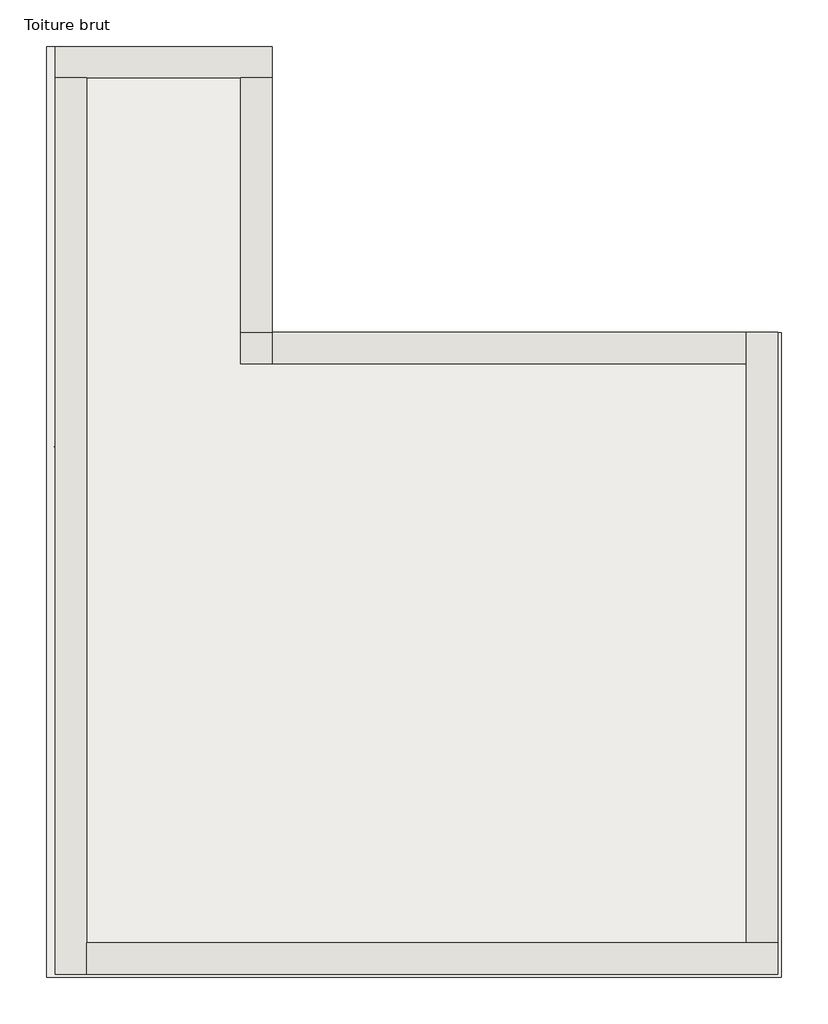
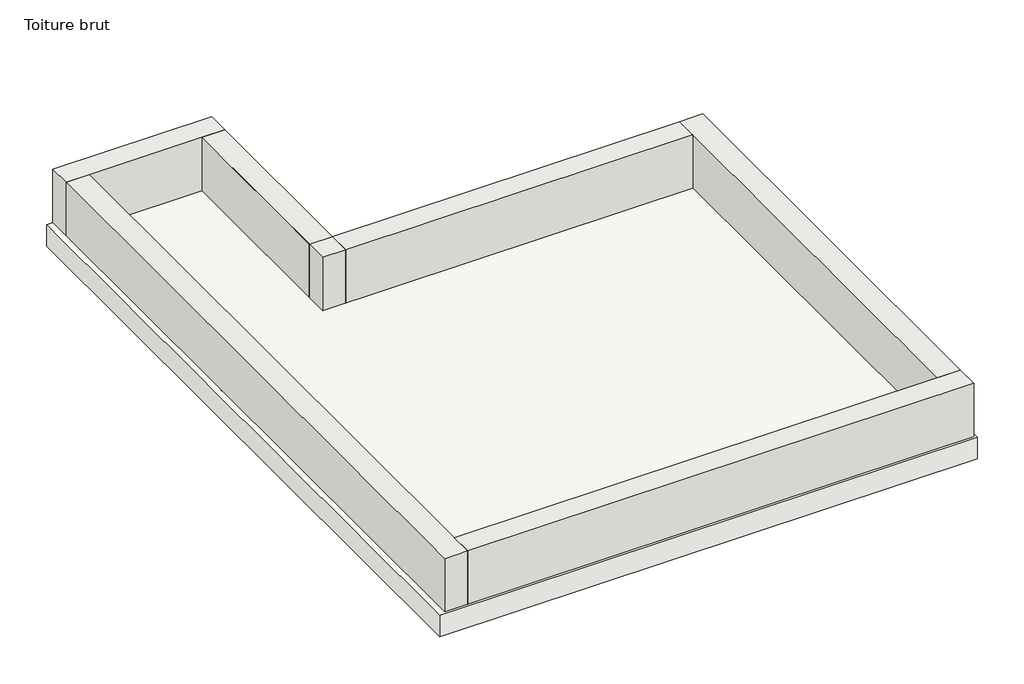
# One storey: 7 walls, 1 slab.
"""IFC4 building model written with IfcOpenShell, lengths in millimetres."""

from ifc_helpers import new_model, si_unit, frame, origin, place, context, project, spatial, polyline, outline, extrude, faceted_brep, element, save

model = new_model("IFC4")

# Units and contexts
model_context = context("Model", 3, world=origin())
ifc_project = project(units=[si_unit("LENGTHUNIT", "METRE", prefix="MILLI")], contexts=[model_context])

# Site, building, storey
site = spatial("IfcSite", under=ifc_project)
building = spatial("IfcBuilding", under=site)
storey = spatial("IfcBuildingStorey", under=building, Name="Toiture brut", Elevation=5410.0)

# Slab
placement = place(None, origin())
element("IfcSlab", 1, ObjectType="Dalla BA 20", at=placement, inside=storey, context=model_context, shape_type="Brep", body=[
    faceted_brep([(-4812.6214092, -828.5605356, 5210.0), (-4812.6214092, -2648.5605356, 5210.0), (-1572.6214092, -2648.5605356, 5210.0), (-1572.6214092, -6548.7020841, 5210.0), (-1572.6214092, -6748.5605356, 5210.0), (-6247.6214092, -6748.5605356, 5210.0), (-6247.6214092, -828.5605356, 5210.0), (-6246.4904447, -828.5605356, 5210.0), (-5012.6214092, -828.5605356, 5210.0), (-6093.4574361, -3373.5605356, 5210.0), (-6146.4904447, -3320.527527, 5210.0), (-6199.5234533, -3373.5605356, 5210.0), (-6146.4904447, -3426.5935442, 5210.0), (-4812.6214092, -2648.5605356, 5410.0), (-4812.6214092, -1028.5605356, 5410.0), (-4812.6214092, -828.5605356, 5410.0), (-6193.4574361, -828.5605356, 5410.0), (-6247.6214092, -828.5605356, 5410.0), (-6247.6214092, -6748.5605356, 5410.0), (-1572.6214092, -6748.5605356, 5410.0), (-1572.6214092, -6548.7020841, 5410.0), (-1572.6214092, -2648.5605356, 5410.0), (-6146.4904447, -3320.527527, 5410.0), (-6093.4574361, -3373.5605356, 5410.0), (-6146.4904447, -3426.5935442, 5410.0), (-6199.5234533, -3373.5605356, 5410.0)], [[[0, 1, 2, 3, 4, 5, 6, 7, 8], [9, 10, 11, 12]], [[13, 14, 15, 16, 17, 18, 19, 20, 21], [22, 23, 24, 25]], [[1, 0, 15, 14, 13]], [[2, 1, 13, 21]], [[4, 3, 2, 21, 20, 19]], [[5, 4, 19, 18]], [[6, 5, 18, 17]], [[0, 8, 7, 6, 17, 16, 15]], [[9, 23, 22, 10]], [[10, 22, 25, 11]], [[11, 25, 24, 12]], [[23, 9, 12, 24]]]),
])

# Walls
element("IfcWall", 2, ObjectType="Bloc à brancher 20 cm", at=placement, inside=storey, context=model_context, shape_type="Brep", body=[
    faceted_brep([(-4812.6214092, -828.5605356, 5410.0), (-6193.4574361, -828.5605356, 5410.0), (-6193.4574361, -828.5605356, 5900.0), (-4812.6214092, -828.5605356, 5900.0), (-4812.6214092, -1028.5605356, 5410.0), (-4812.6214092, -1028.5605356, 5900.0), (-5012.6214092, -1028.5605356, 5900.0), (-5993.4574361, -1028.5605356, 5900.0), (-6193.4574361, -1028.5605356, 5900.0), (-6193.4574361, -1028.5605356, 5410.0), (-5993.4574361, -1028.5605356, 5410.0), (-5012.6214092, -1028.5605356, 5410.0)], [[[0, 1, 2, 3]], [[4, 5, 6, 7, 8, 9, 10, 11]], [[1, 0, 4, 11, 10, 9]], [[3, 2, 8, 7, 6, 5]], [[2, 1, 9, 8]], [[0, 3, 5, 4]]]),
])
element("IfcWall", 3, ObjectType="Bloc à brancher 20 cm", at=placement, inside=storey, context=model_context, shape_type="Brep", body=[
    faceted_brep([(-6193.4574361, -1028.5605356, 5410.0), (-6193.4574361, -6728.5605356, 5410.0), (-6193.4574361, -6728.5605356, 5900.0), (-6193.4574361, -1028.5605356, 5900.0), (-5993.4574361, -1028.5605356, 5410.0), (-5993.4574361, -1028.5605356, 5900.0), (-5993.4574361, -6528.5605356, 5900.0), (-5993.4574361, -6728.5605356, 5900.0), (-5993.4574361, -6728.5605356, 5410.0), (-5993.4574361, -6528.5605356, 5410.0)], [[[0, 1, 2, 3]], [[4, 5, 6, 7, 8, 9]], [[1, 0, 4, 9, 8]], [[3, 2, 7, 6, 5]], [[0, 3, 5, 4]], [[2, 1, 8, 7]]]),
])
element("IfcWall", 4, ObjectType="Bloc à brancher 20 cm", at=placement, inside=storey, context=model_context, shape_type="Brep", body=[
    faceted_brep([(-5993.4574361, -6728.5605356, 5410.0), (-1593.4574361, -6728.5605356, 5410.0), (-1593.4574361, -6728.5605356, 5900.0), (-5993.4574361, -6728.5605356, 5900.0), (-5993.4574361, -6528.5605356, 5410.0), (-5993.4574361, -6528.5605356, 5900.0), (-1793.4574361, -6528.5605356, 5900.0), (-1593.4574361, -6528.5605356, 5900.0), (-1593.4574361, -6528.5605356, 5410.0), (-1793.4574361, -6528.5605356, 5410.0)], [[[0, 1, 2, 3]], [[4, 5, 6, 7, 8, 9]], [[1, 0, 4, 9, 8]], [[3, 2, 7, 6, 5]], [[0, 3, 5, 4]], [[2, 1, 8, 7]]]),
])
element("IfcWall", 5, ObjectType="Bloc à brancher 20 cm", at=placement, inside=storey, context=model_context, shape_type="Brep", body=[
    faceted_brep([(-1593.4574361, -6528.5605356, 5410.0), (-1593.4574361, -2846.164631, 5410.0), (-1593.4574361, -2646.164631, 5410.0), (-1593.4574361, -2646.164631, 5900.0), (-1593.4574361, -6528.5605356, 5900.0), (-1793.4574361, -6528.5605356, 5410.0), (-1793.4574361, -6528.5605356, 5900.0), (-1793.4574361, -2846.164631, 5900.0), (-1793.4574361, -2646.164631, 5900.0), (-1793.4574361, -2646.164631, 5410.0), (-1793.4574361, -2846.164631, 5410.0), (-1766.4904447, -2646.164631, 5410.0)], [[[0, 1, 2, 3, 4]], [[5, 6, 7, 8, 9, 10]], [[2, 1, 0, 5, 10, 9, 11]], [[4, 3, 8, 7, 6]], [[0, 4, 6, 5]], [[3, 2, 11, 9, 8]]]),
])
element("IfcWall", 6, ObjectType="Bloc à brancher 20 cm", at=placement, inside=storey, context=model_context, shape_type="SweptSolid", body=[
    extrude(outline(polyline([(-4812.6214092, -1028.5605356), (-4812.6214092, -2646.164631), (-5012.6214092, -2646.164631), (-5012.6214092, -1028.5605356), (-4812.6214092, -1028.5605356)])), frame((0.0, 0.0, 5410.0), z_axis=(0.0, 0.0, 1.0), x_axis=(1.0, 0.0, 0.0)), (0.0, 0.0, 1.0), 490.0),
])
element("IfcWall", 7, ObjectType="Bloc à brancher 20 cm", at=placement, inside=storey, context=model_context, shape_type="SweptSolid", body=[
    extrude(outline(polyline([(-4812.6214092, -2646.164631), (-1793.4574361, -2646.164631), (-1793.4574361, -2846.164631), (-4812.6214092, -2846.164631), (-4812.6214092, -2646.164631)])), frame((0.0, 0.0, 5410.0), z_axis=(0.0, 0.0, 1.0), x_axis=(1.0, 0.0, 0.0)), (0.0, 0.0, 1.0), 490.0),
])
element("IfcWall", 8, ObjectType="Bloc à brancher 20 cm", at=placement, inside=storey, context=model_context, shape_type="Brep", body=[
    faceted_brep([(-5012.6214092, -1028.5605356, 5410.0), (-5012.6214092, -2846.164631, 5410.0), (-5012.6214092, -2846.164631, 5900.0), (-5012.6214092, -1028.5605356, 5900.0), (-4812.6214092, -1028.5605356, 5410.0), (-4812.6214092, -1028.5605356, 5900.0), (-4812.6214092, -2646.164631, 5900.0), (-4812.6214092, -2846.164631, 5900.0), (-4812.6214092, -2846.164631, 5410.0), (-4812.6214092, -2646.164631, 5410.0)], [[[0, 1, 2, 3]], [[4, 5, 6, 7, 8, 9]], [[1, 0, 4, 9, 8]], [[3, 2, 7, 6, 5]], [[0, 3, 5, 4]], [[2, 1, 8, 7]]]),
])

save(model, "model.ifc")

# Revit data of these elements
# Type "Dalla BA 20"
#   Function = 0
#   Layers, outside or top first: 0.200 m "Béton - Coulé sur place - Béton25" (function 1)
# Type "Bloc à brancher 20 cm"
#   Layers, outside or top first: 0.025 m "Blocs béton manufacturés" (function 1); 0.150 m "Béton - Coulé sur place - Béton25" (function 1); 0.025 m "Blocs béton manufacturés" (function 1)
# Element 1 (IfcSlab, "Dalla BA 20")
#   Height Offset From Level = 0.000 m
#   built-in parameter 1001954 = 1
#   Phase Created = Nouvelle construction
#   Materials on its faces: "Béton - Coulé sur place - Béton25"
# Elements 2, 3, 4, 5, 8 (IfcWall, "Bloc à brancher 20 cm")
#   Top Offset = 0.000 m
#   Base Offset = 0.000 m
#   wall height = 0.490 m
#   Phase Created = Nouvelle construction
#   Base Constraint = Toiture brut
#   Top Constraint = As acrotère TOITURE
#   Materials on its faces: "Blocs béton manufacturés", "Mur par défaut"
# Elements 6, 7 (IfcWall, "Bloc à brancher 20 cm")
#   Top Offset = 0.000 m
#   Base Offset = 0.000 m
#   wall height = 0.490 m
#   Phase Created = Nouvelle construction
#   Base Constraint = Toiture brut
#   Top Constraint = As acrotère TOITURE
#   Materials on its faces: "Mur par défaut", "Blocs béton manufacturés"
# Materials
#   "Béton - Coulé sur place - Béton25": class "Béton", colour RGB 192 192 192, transparency 0, Cost = 0
#   "Blocs béton manufacturés": class "Maçonnerie", colour RGB 152 154 138, transparency 0, Description = "Blocs béton manufacturés", Cost = 0
#   "Mur par défaut": class "Divers", colour RGB 128 128 128, transparency 0, Cost = 0
